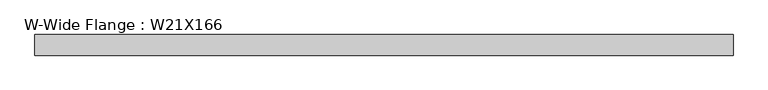
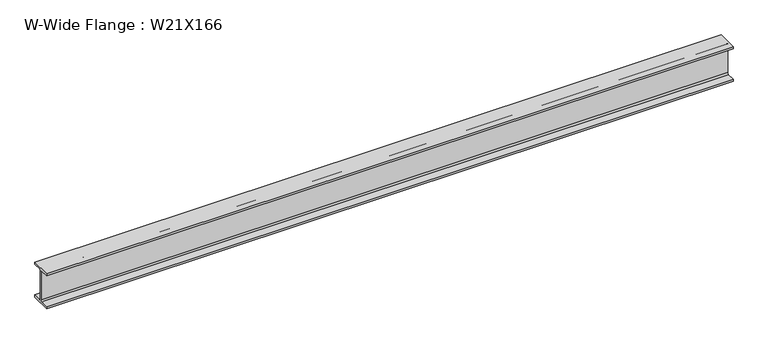
"""IFC4 building model written with IfcOpenShell, lengths in millimetres: beam geometry, W-Wide Flange : W21X166."""

from ifc_helpers import new_model, si_unit, point, frame, frame_2d, origin, place, context, project, spatial, polyline, circle_curve, trimmed, segment, composite_curve, outline, extrude, source, transform, mapped, element, save


def w_wide_flange_w21x166_0aa46e18(model_context):
    return source(origin(), model_context, "Body", "SweptSolid", [
        extrude(outline(composite_curve([segment(polyline([(157.48, -251.206), (157.48, -285.75), (-157.48, -285.75), (-157.48, -251.206), (-32.131, -251.206)]), True, "CONTINUOUS"), segment(trimmed(circle_curve(frame_2d((-32.131, -228.6)), 22.606), [point((-32.131, -251.206))], [point((-9.525, -228.6))], True, "CARTESIAN"), True, "CONTINUOUS"), segment(polyline([(-9.525, -228.6), (-9.525, 228.6)]), True, "CONTINUOUS"), segment(trimmed(circle_curve(frame_2d((-32.131, 228.6)), 22.606), [point((-9.525, 228.6))], [point((-32.131, 251.206))], True, "CARTESIAN"), True, "CONTINUOUS"), segment(polyline([(-32.131, 251.206), (-157.48, 251.206), (-157.48, 285.75), (157.48, 285.75), (157.48, 251.206), (32.131, 251.206)]), True, "CONTINUOUS"), segment(trimmed(circle_curve(frame_2d((32.131, 228.6)), 22.606), [point((32.131, 251.206))], [point((9.525, 228.6))], True, "CARTESIAN"), True, "CONTINUOUS"), segment(polyline([(9.525, 228.6), (9.525, -228.6)]), True, "CONTINUOUS"), segment(trimmed(circle_curve(frame_2d((32.131, -228.6)), 22.606), [point((9.525, -228.6))], [point((32.131, -251.206))], True, "CARTESIAN"), True, "CONTINUOUS"), segment(polyline([(32.131, -251.206), (157.48, -251.206)]), True, "CONTINUOUS")], self_intersect=False)), frame((-5422.8338829, 0.0, 0.0), z_axis=(1.0, 0.0, 0.0), x_axis=(0.0, 1.0, 0.0)), (0.0, 0.0, 1.0), 10659.8214497),
    ])


if __name__ == "__main__":
    model = new_model("IFC4")
    model_context = context("Model", 3, world=origin())
    ifc_project = project(units=[si_unit("LENGTHUNIT", "METRE", prefix="MILLI")], contexts=[model_context])
    site = spatial("IfcSite", under=ifc_project)
    building = spatial("IfcBuilding", under=site)
    placement = place(None, origin())
    w_wide_flange_w21x166_shape = w_wide_flange_w21x166_0aa46e18(model_context)
    element("IfcBeam", 1, ObjectType="W-Wide Flange : W21X166", at=placement, inside=building, context=model_context, shape_type="MappedRepresentation", body=[
        mapped(w_wide_flange_w21x166_shape, transform((0.0, 0.0, 0.0), x_axis=(1.0, 0.0, 0.0), y_axis=(0.0, 1.0, 0.0), z_axis=(0.0, 0.0, 1.0))),
    ])
    save(model, "model.ifc")

# Revit data of these elements
# Type "W-Wide Flange : W21X166"
#   Assembly Code = "B10"
#   W = 166
#   Length [instance default] = 5' - 0"
#   bf = 1' - 0.4"
#   d = 1' - 10 1/2"
#   k = 0' - 2 1/4"
#   k2 = 0' - 0.89"
#   tf = 0' - 1.36"
#   tw = 0' - 0 3/4"
#   A = 0.338889 SF
#   Structural Material [instance default] = Steel ASTM A992
# Element 1 (IfcBeam, "W-Wide Flange : W21X166")
#   Structural Material = Steel
#   Materials on its faces: "Steel"
# Materials
#   "Steel ASTM A992": class "Metal", colour RGB 199 199 199, transparency 0, Description = "Structural steel 50ksi", Cost = 0
#   "Steel": class "Metal", colour RGB 118 118 114, transparency 0, Description = "Steel, mill finish", Cost = 0
